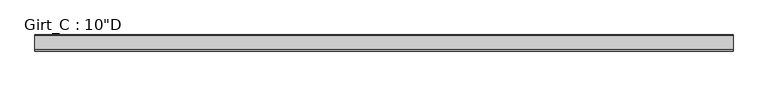
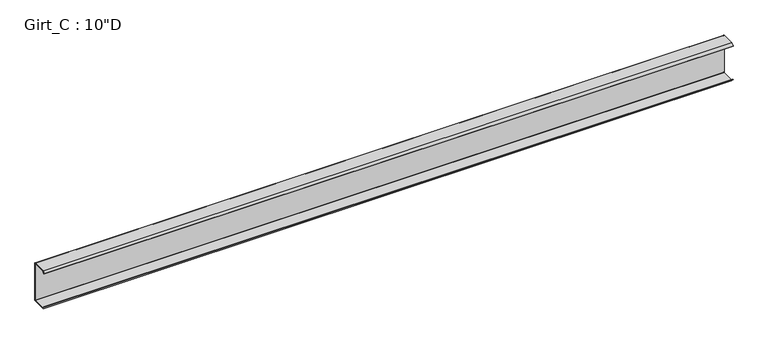
"""IFC4 building model written with IfcOpenShell, lengths in millimetres: beam geometry."""

from ifc_helpers import new_model, si_unit, point, frame, frame_2d, origin, place, context, project, spatial, polyline, circle_curve, trimmed, segment, composite_curve, outline, extrude, source, transform, mapped, element, save


def beam_3b9f553c(model_context):
    return source(origin(), model_context, "Body", "SweptSolid", [
        extrude(outline(composite_curve([segment(polyline([(-87.5109375, 127.0), (-3.3734375, 127.0)]), True, "CONTINUOUS"), segment(trimmed(circle_curve(frame_2d((-3.3734375, 122.2375)), 4.7625), [point((-3.3734375, 127.0))], [point((1.3890625, 122.2375))], False, "CARTESIAN"), True, "CONTINUOUS"), segment(polyline([(1.3890625, 122.2375), (1.3890625, -122.2375)]), True, "CONTINUOUS"), segment(trimmed(circle_curve(frame_2d((-3.3734375, -122.2375)), 4.7625), [point((1.3890625, -122.2375))], [point((-3.3734375, -127.0))], False, "CARTESIAN"), True, "CONTINUOUS"), segment(polyline([(-3.3734375, -127.0), (-87.5109375, -127.0), (-99.7792647, -112.379177), (-97.6510975, -110.5934327), (-86.2154765, -124.221875), (-3.2694106, -124.221875)]), True, "CONTINUOUS"), segment(trimmed(circle_curve(frame_2d((-3.3748024, -122.2389339)), 1.9857399), [point((-3.2694106, -124.221875))], [point((-1.3890625, -122.2389339))], True, "CARTESIAN"), True, "CONTINUOUS"), segment(polyline([(-1.3890625, -122.2389339), (-1.3890625, 122.2381931)]), True, "CONTINUOUS"), segment(trimmed(circle_curve(frame_2d((-3.3741066, 122.2381931)), 1.9850441), [point((-1.3890625, 122.2381931))], [point((-3.3005807, 124.221875))], True, "CARTESIAN"), True, "CONTINUOUS"), segment(polyline([(-3.3005807, 124.221875), (-86.2154765, 124.221875), (-97.6278742, 110.621109), (-99.7560415, 112.4068534), (-87.5109375, 127.0)]), True, "CONTINUOUS")], self_intersect=False)), frame((-2199.894, 0.0, 0.0), z_axis=(1.0, 0.0, 0.0), x_axis=(0.0, 1.0, 0.0)), (0.0, 0.0, 1.0), 4368.038),
    ])


if __name__ == "__main__":
    model = new_model("IFC4")
    model_context = context("Model", 3, world=origin())
    ifc_project = project(units=[si_unit("LENGTHUNIT", "METRE", prefix="MILLI")], contexts=[model_context])
    site = spatial("IfcSite", under=ifc_project)
    building = spatial("IfcBuilding", under=site)
    placement = place(None, origin())
    beam_shape = beam_3b9f553c(model_context)
    element("IfcBeam", 1, ObjectType="Girt_C : 10\"D", at=placement, inside=building, context=model_context, shape_type="MappedRepresentation", body=[
        mapped(beam_shape, transform((0.0, 0.0, 0.0), x_axis=(1.0, 0.0, 0.0), y_axis=(0.0, 1.0, 0.0), z_axis=(0.0, 0.0, 1.0))),
    ])
    save(model, "model.ifc")

# Revit data of these elements
# Type "Girt_C : 10\"D"
#   half leg = 0' - 1 3/4"
#   Web_Thickness = 0' - 0 7/64"
#   Length [instance default] = 10' - 0"
#   Leg_1 = 0' - 3 1/2"
#   Height = 0' - 10"
#   Structural Material [instance default] = none
# Element 1 (IfcBeam, "Girt_C : 10\"D")
#   Structural Material = STRUCTURAL STEEL - SEE STRUCT. DWGS
#   Materials on its faces: "STRUCTURAL STEEL - SEE STRUCT. DWGS"
# Materials
#   "STRUCTURAL STEEL - SEE STRUCT. DWGS": class "Metal", colour RGB 137 146 153, transparency 0, Description = "Steel, mill finish", Cost = 0
